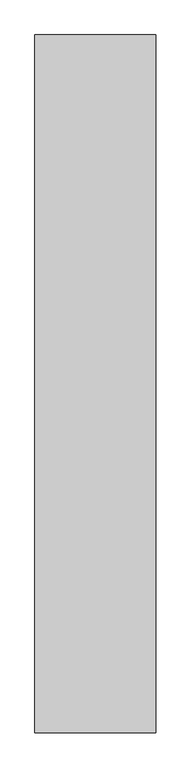
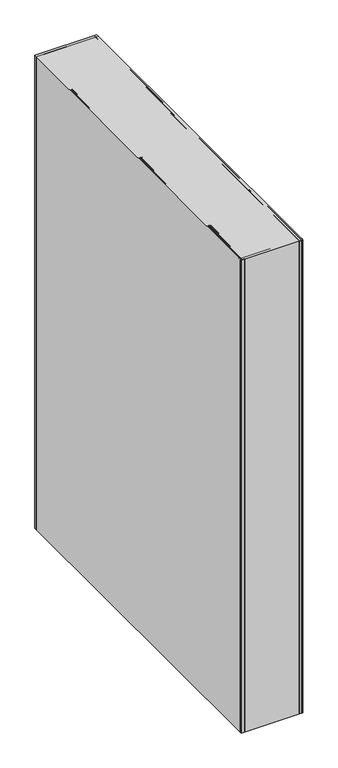
"""IFC4 building model written with IfcOpenShell, lengths in millimetres: beam geometry, LF02ZBK001_DIKE WALL_RC : Dike_Thk.260_EW1."""

from ifc_helpers import new_model, si_unit, origin, origin_with_axes, place, context, project, spatial, polyline, outline, extrude, source, transform, mapped, element, save


def beam_3de7345f(model_context):
    return source(origin(), model_context, "Body", "SweptSolid", [
        extrude(outline(polyline([(130.0, -750.0), (-130.0, -750.0), (-130.0, 750.0), (130.0, 750.0), (130.0, -750.0)])), origin_with_axes(), (0.0, 0.0, 1.0), 2100.0),
        extrude(outline(polyline([(-130.0, -735.0), (-130.0, -734.0), (130.0, -734.0), (130.0, -735.0), (-130.0, -735.0)])), origin_with_axes(), (0.0, 0.0, 1.0), 2100.0),
        extrude(outline(polyline([(-130.0, -740.0), (-130.0, -739.0), (130.0, -739.0), (130.0, -740.0), (-130.0, -740.0)])), origin_with_axes(), (0.0, 0.0, 1.0), 2100.0),
        extrude(outline(polyline([(-130.0, -745.0), (-130.0, -744.0), (130.0, -744.0), (130.0, -745.0), (-130.0, -745.0)])), origin_with_axes(), (0.0, 0.0, 1.0), 2100.0),
        extrude(outline(polyline([(-130.0, 735.0), (130.0, 735.0), (130.0, 734.0), (-130.0, 734.0), (-130.0, 735.0)])), origin_with_axes(), (0.0, 0.0, 1.0), 2100.0),
        extrude(outline(polyline([(-130.0, 740.0), (130.0, 740.0), (130.0, 739.0), (-130.0, 739.0), (-130.0, 740.0)])), origin_with_axes(), (0.0, 0.0, 1.0), 2100.0),
        extrude(outline(polyline([(-130.0, 745.0), (130.0, 745.0), (130.0, 744.0), (-130.0, 744.0), (-130.0, 745.0)])), origin_with_axes(), (0.0, 0.0, 1.0), 2100.0),
        extrude(outline(polyline([(114.0, 750.0), (115.0, 750.0), (115.0, -750.0), (114.0, -750.0), (114.0, 750.0)])), origin_with_axes(), (0.0, 0.0, 1.0), 2100.0),
        extrude(outline(polyline([(119.0, 750.0), (120.0, 750.0), (120.0, -750.0), (119.0, -750.0), (119.0, 750.0)])), origin_with_axes(), (0.0, 0.0, 1.0), 2100.0),
        extrude(outline(polyline([(124.0, 750.0), (125.0, 750.0), (125.0, -750.0), (124.0, -750.0), (124.0, 750.0)])), origin_with_axes(), (0.0, 0.0, 1.0), 2100.0),
        extrude(outline(polyline([(-114.0, 750.0), (-114.0, -750.0), (-115.0, -750.0), (-115.0, 750.0), (-114.0, 750.0)])), origin_with_axes(), (0.0, 0.0, 1.0), 2100.0),
        extrude(outline(polyline([(-119.0, 750.0), (-119.0, -750.0), (-120.0, -750.0), (-120.0, 750.0), (-119.0, 750.0)])), origin_with_axes(), (0.0, 0.0, 1.0), 2100.0),
        extrude(outline(polyline([(-124.0, 750.0), (-124.0, -750.0), (-125.0, -750.0), (-125.0, 750.0), (-124.0, 750.0)])), origin_with_axes(), (0.0, 0.0, 1.0), 2100.0),
    ])


if __name__ == "__main__":
    model = new_model("IFC4")
    model_context = context("Model", 3, world=origin())
    ifc_project = project(units=[si_unit("LENGTHUNIT", "METRE", prefix="MILLI")], contexts=[model_context])
    site = spatial("IfcSite", under=ifc_project)
    building = spatial("IfcBuilding", under=site)
    placement = place(None, origin())
    beam_shape = beam_3de7345f(model_context)
    element("IfcBeam", 1, ObjectType="LF02ZBK001_DIKE WALL_RC : Dike_Thk.260_EW1", at=placement, inside=building, context=model_context, shape_type="MappedRepresentation", body=[
        mapped(beam_shape, transform((0.0, 0.0, 0.0), x_axis=(1.0, 0.0, 0.0), y_axis=(0.0, 1.0, 0.0), z_axis=(0.0, 0.0, 1.0))),
    ])
    save(model, "model.ifc")

# Revit data of these elements
# Type "LF02ZBK001_DIKE WALL_RC : Dike_Thk.260_EW1"
#   Dike_thk = 260 mm
#   Dike_Length [instance default] = 3000 mm
#   Dike_Hight = 2100 mm
#   c2_visible = yes
#   c3_material [instance default] = none
#   c2_material 3 [instance default] = none
#   c2_material 2 [instance default] = none
#   c2_material 1 [instance default] = none
#   c1_material [instance default] = none
#   Default Elevation = 0
# Element 1 (IfcBeam, "LF02ZBK001_DIKE WALL_RC : Dike_Thk.260_EW1")
#   Dike_Length = 1500 mm
